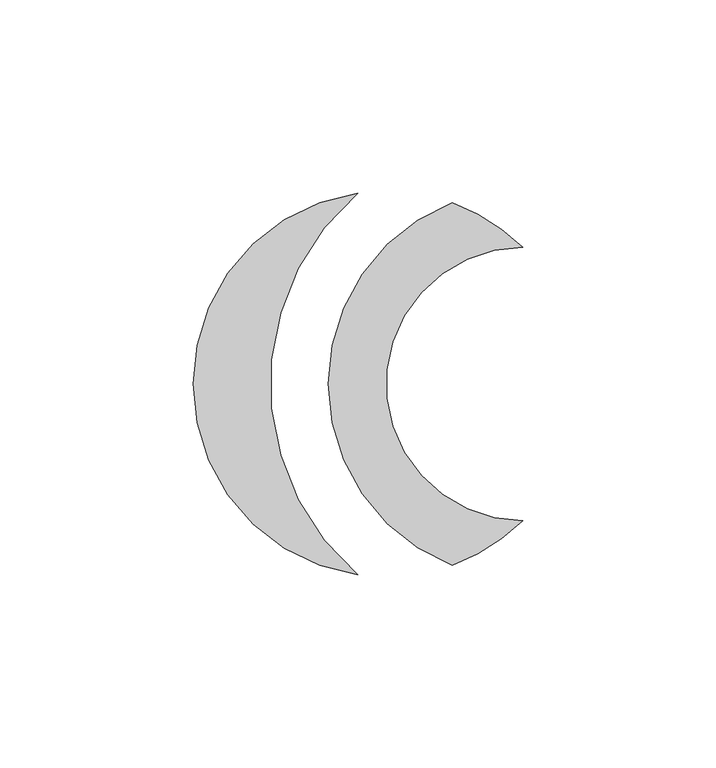
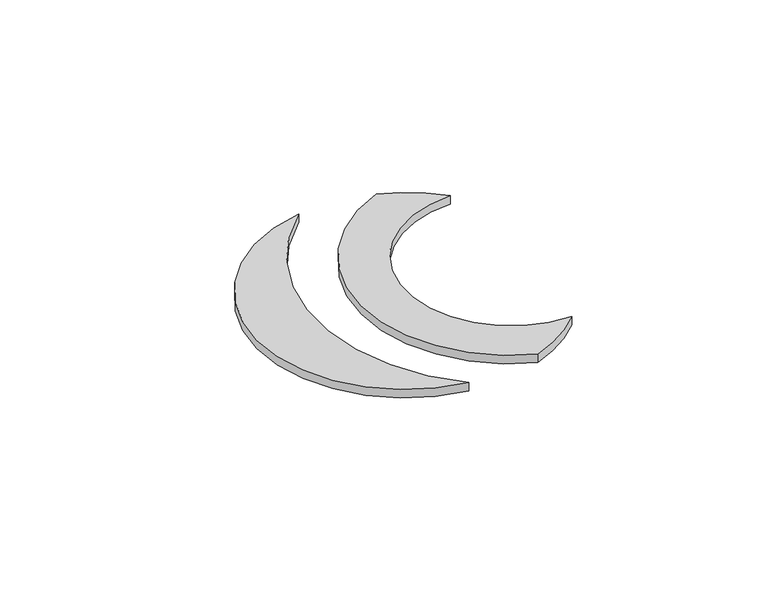
"""IFC4 building model written with IfcOpenShell, lengths in millimetres: proxy geometry, TSP Dimmers : TSP Dimmers."""

from ifc_helpers import new_model, si_unit, point, frame_2d, origin, origin_with_axes, origin_2d, place, context, project, spatial, circle_curve, trimmed, segment, composite_curve, outline, extrude, source, transform, mapped, element, save


def electrical_fixtures_9bf589c6(model_context):
    return source(origin(), model_context, "Body", "SweptSolid", [
        extrude(outline(composite_curve([segment(trimmed(circle_curve(origin_2d(), 50.0), [point((17.1733585, 46.9582342))], [point((35.3553391, 35.3553391))], False, "CARTESIAN"), True, "CONTINUOUS"), segment(trimmed(circle_curve(frame_2d((35.3553391, 0.0)), 35.3553391), [point((35.3553391, 35.3553391))], [point((35.3553391, -35.3553391))], True, "CARTESIAN"), True, "CONTINUOUS"), segment(trimmed(circle_curve(origin_2d(), 50.0), [point((35.3553391, -35.3553391))], [point((17.1733585, -46.9582342))], False, "CARTESIAN"), True, "CONTINUOUS"), segment(trimmed(circle_curve(frame_2d((35.3553391, 0.0)), 50.3553391), [point((17.1733585, -46.9582342))], [point((17.1733585, 46.9582342))], False, "CARTESIAN"), True, "CONTINUOUS")], self_intersect=False)), origin_with_axes(), (0.0, 0.0, 1.0), 3.0),
        extrude(outline(composite_curve([segment(trimmed(circle_curve(frame_2d((35.3553391, 0.0)), 65.3553391), [point((-7.372583, 49.4534632))], [point((-7.372583, -49.4534632))], True, "CARTESIAN"), True, "CONTINUOUS"), segment(trimmed(circle_curve(origin_2d(), 50.0), [point((-7.372583, -49.4534632))], [point((-7.372583, 49.4534632))], False, "CARTESIAN"), True, "CONTINUOUS")], self_intersect=False)), origin_with_axes(), (0.0, 0.0, 1.0), 3.0),
    ])


if __name__ == "__main__":
    model = new_model("IFC4")
    model_context = context("Model", 3, world=origin())
    ifc_project = project(units=[si_unit("LENGTHUNIT", "METRE", prefix="MILLI")], contexts=[model_context])
    site = spatial("IfcSite", under=ifc_project)
    building = spatial("IfcBuilding", under=site)
    placement = place(None, origin())
    electrical_fixtures_shape = electrical_fixtures_9bf589c6(model_context)
    element("IfcBuildingElementProxy", 1, Name="TSP Dimmers : TSP Dimmers", ObjectType="TSP Dimmers : TSP Dimmers", at=placement, inside=building, context=model_context, shape_type="MappedRepresentation", body=[
        mapped(electrical_fixtures_shape, transform((0.0, 0.0, 0.0), x_axis=(1.0, 0.0, 0.0), y_axis=(0.0, 1.0, 0.0), z_axis=(0.0, 0.0, 1.0))),
    ])
    save(model, "model.ifc")

# Revit data of these elements
# Type "TSP Dimmers : TSP Dimmers"
#   Model = "TSP_ELECDIMS"
#   Default Elevation = 0
# Element 1 (IfcBuildingElementProxy, "TSP Dimmers : TSP Dimmers")
#   Materials on its faces: "Plastic, Opaque Black"
# Materials
#   "Plastic, Opaque Black": class "Plastic", colour RGB 0 0 0, transparency 0.7, Description = "Plastic, generic, opaque black", Cost = 0
